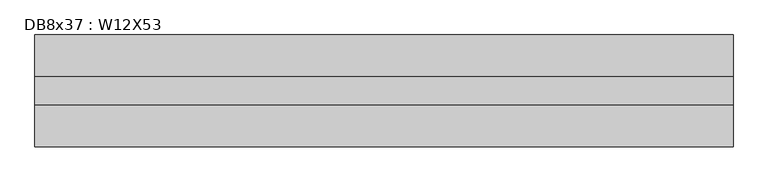
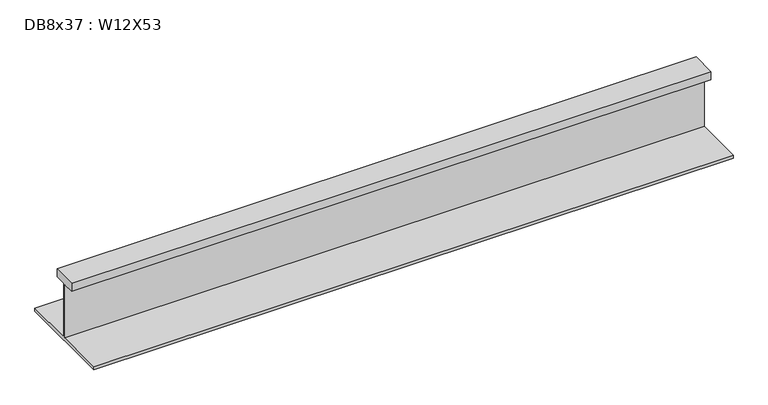
"""IFC4 building model written with IfcOpenShell, lengths in millimetres: beam geometry, DB8x37 : W12X53."""

from ifc_helpers import new_model, si_unit, frame, origin, place, context, project, spatial, polyline, outline, extrude, source, transform, mapped, element, save


def db8x37_w12x53_dbe42cc9(model_context):
    return source(origin(), model_context, "Body", "SweptSolid", [
        extrude(outline(polyline([(38.1, 145.415), (38.1, 120.015), (2.921, 120.015), (2.921, -48.4505), (152.4, -48.4505), (152.4, -58.1025), (-152.4, -58.1025), (-152.4, -48.4505), (-2.921, -48.4505), (-2.921, 120.015), (-38.1, 120.015), (-38.1, 145.415), (38.1, 145.415)])), frame((-914.4, 0.0, 0.0), z_axis=(1.0, 0.0, 0.0), x_axis=(0.0, 1.0, 0.0)), (0.0, 0.0, 1.0), 1905.0),
    ])


if __name__ == "__main__":
    model = new_model("IFC4")
    model_context = context("Model", 3, world=origin())
    ifc_project = project(units=[si_unit("LENGTHUNIT", "METRE", prefix="MILLI")], contexts=[model_context])
    site = spatial("IfcSite", under=ifc_project)
    building = spatial("IfcBuilding", under=site)
    placement = place(None, origin())
    db8x37_w12x53_shape = db8x37_w12x53_dbe42cc9(model_context)
    element("IfcBeam", 1, ObjectType="DB8x37 : W12X53", at=placement, inside=building, context=model_context, shape_type="MappedRepresentation", body=[
        mapped(db8x37_w12x53_shape, transform((0.0, 0.0, 0.0), x_axis=(1.0, 0.0, 0.0), y_axis=(0.0, 1.0, 0.0), z_axis=(0.0, 0.0, 1.0))),
    ])
    save(model, "model.ifc")

# Revit data of these elements
# Type "DB8x37 : W12X53"
#   Assembly Code = "B10"
#   W = 53
#   Length [instance default] = 5' - 0"
#   bf = 0' - 10"
#   d = 1' - 0.1"
#   k = 0' - 1 3/8"
#   k2 = 0' - 0.8"
#   tf = 0' - 0.575"
#   tw = 0' - 0.345"
#   A = 0.108333 SF
#   Structural Material [instance default] = Steel ASTM A992
# Element 1 (IfcBeam, "DB8x37 : W12X53")
#   Materials on its faces: "Steel ASTM A992"
# Materials
#   "Steel ASTM A992": class "Metal", colour RGB 199 199 199, transparency 0, Description = "Structural steel 50ksi", Cost = 0
